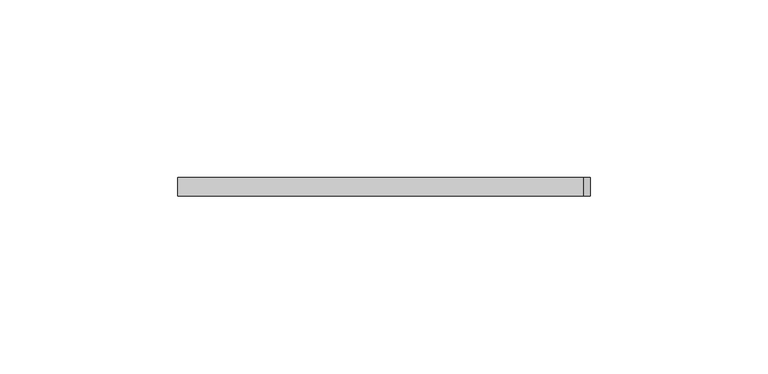
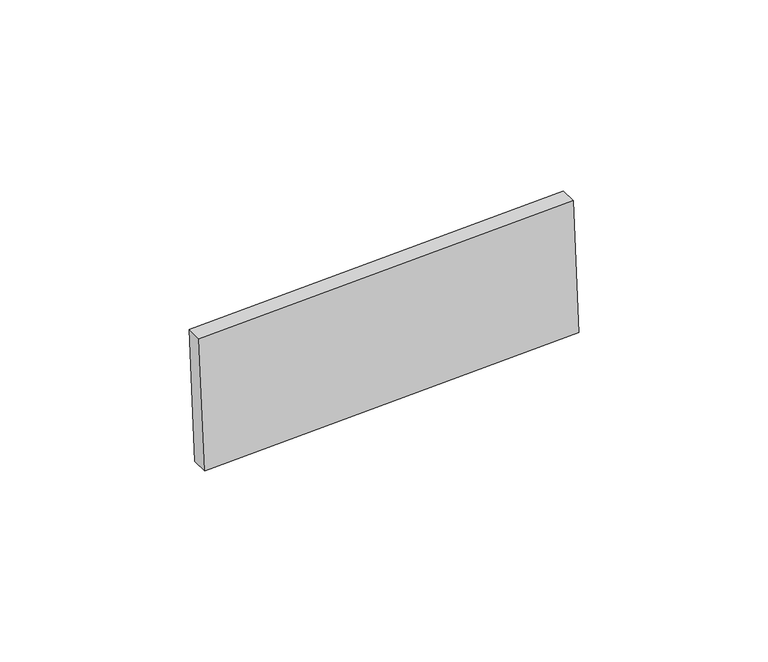
"""IFC4 building model written with IfcOpenShell, lengths in millimetres: proxy geometry, Inner panel:Inner panel:1:Inner panel:1 : Inner panel:Inner panel:300324:2:Inner panel:1:Inner panel:1 : Inner panel:Inner panel:300324:2 : Inner panel:Inner panel:1:Inner panel:1 : Inner panel:Inner panel:300324:300043:150 : Inner panel:Inner panel:1:Inner panel:1 : Inner panel:Inner panel:300324:2:Inner panel:1:Inner panel:1 : Inner panel:Inner panel:300324:2 : Inner panel:Inner panel:1:Inner panel:1 : Inner panel:Inner panel:300324:300043:308120."""

from ifc_helpers import new_model, si_unit, frame, origin, place, context, project, spatial, polyline, outline, extrude, source, transform, mapped, element, save


def generic_models_cbd0968f(model_context):
    return source(origin(), model_context, "Body", "SweptSolid", [
        extrude(outline(polyline([(0.0, -114.3), (0.0, 0.0), (5.2138089, 0.0), (5.2138089, -114.3), (0.0, -114.3)])), frame((560425.2415304, -578534.9848948, 3954.8593664), z_axis=(-0.04163054471216399, 0.0, 0.9991330730923527), x_axis=(0.0, -1.0, 0.0)), (0.0, 0.0, 1.0), 43.2233908),
    ])


if __name__ == "__main__":
    model = new_model("IFC4")
    model_context = context("Model", 3, world=origin())
    ifc_project = project(units=[si_unit("LENGTHUNIT", "METRE", prefix="MILLI")], contexts=[model_context])
    site = spatial("IfcSite", under=ifc_project)
    building = spatial("IfcBuilding", under=site)
    placement = place(None, origin())
    generic_models_shape = generic_models_cbd0968f(model_context)
    element("IfcBuildingElementProxy", 1, Name="Inner panel:Inner panel:1:Inner panel:1 : Inner panel:Inner panel:300324:2:Inner panel:1:Inner panel:1 : Inner panel:Inner panel:300324:2 : Inner panel:Inner panel:1:Inner panel:1 : Inner panel:Inner panel:300324:300043:150 : Inner panel:Inner panel:1:Inner panel:1 : Inner panel:Inner panel:300324:2:Inner panel:1:Inner panel:1 : Inner panel:Inner panel:300324:2 : Inner panel:Inner panel:1:Inner panel:1 : Inner panel:Inner panel:300324:300043:308120", ObjectType="Inner panel:Inner panel:1:Inner panel:1 : Inner panel:Inner panel:300324:2:Inner panel:1:Inner panel:1 : Inner panel:Inner panel:300324:2 : Inner panel:Inner panel:1:Inner panel:1 : Inner panel:Inner panel:300324:300043:150 : Inner panel:Inner panel:1:Inner panel:1 : Inner panel:Inner panel:300324:2:Inner panel:1:Inner panel:1 : Inner panel:Inner panel:300324:2 : Inner panel:Inner panel:1:Inner panel:1 : Inner panel:Inner panel:300324:300043:308120", at=placement, inside=building, context=model_context, shape_type="MappedRepresentation", body=[
        mapped(generic_models_shape, transform((0.0, 0.0, 0.0), x_axis=(1.0, 0.0, 0.0), y_axis=(0.0, 1.0, 0.0), z_axis=(0.0, 0.0, 1.0))),
    ])
    save(model, "model.ifc")

# Revit data of these elements
# Type "Inner panel:Inner panel:1:Inner panel:1 : Inner panel:Inner panel:300324:2:Inner panel:1:Inner panel:1 : Inner panel:Inner panel:300324:2 : Inner panel:Inner panel:1:Inner panel:1 : Inner panel:Inner panel:300324:300043:150 : Inner panel:Inner panel:1:Inner panel:1 : Inner panel:Inner panel:300324:2:Inner panel:1:Inner panel:1 : Inner panel:Inner panel:300324:2 : Inner panel:Inner panel:1:Inner panel:1 : Inner panel:Inner panel:300324:300043:308120"
#   NameOverride = "Inner panel:Inner panel:1:Inner panel:1 : Inner panel:Inner panel:300324:2:Inner panel:1:Inner panel:1 : Inner panel:Inner panel:300324:2 : Inner panel:Inner panel:1:Inner panel:1 : Inner panel:Inner panel:300324:300043:308120"
#   ObjectTypeOverride = "Inner panel:1:Inner panel:1 : Inner panel:Inner panel:300324:2 : Inner panel:Inner panel:1:Inner panel:1 : Inner panel:Inner panel:300324:300043"
#   Reference = "Inner panel"
#   Tag = "308120"
# Element 1 (IfcBuildingElementProxy, "Inner panel:Inner panel:1:Inner panel:1 : Inner panel:Inner panel:300324:2:Inner panel:1:Inner panel:1 : Inner panel:Inner panel:300324:2 : Inner panel:Inner panel:1:Inner panel:1 : Inner panel:Inner panel:300324:300043:150 : Inner panel:Inner panel:1:Inner panel:1 : Inner panel:Inner panel:300324:2:Inner panel:1:Inner panel:1 : Inner panel:Inner panel:300324:2 : Inner panel:Inner panel:1:Inner panel:1 : Inner panel:Inner panel:300324:300043:308120")
#   Materials on its faces: "SLIDING CLIP"
# Materials
#   "SLIDING CLIP": class "Generic", colour RGB 120 120 120, transparency 0, Cost = 0
